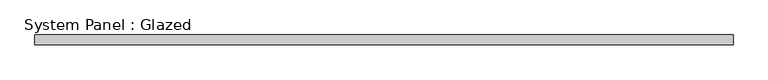
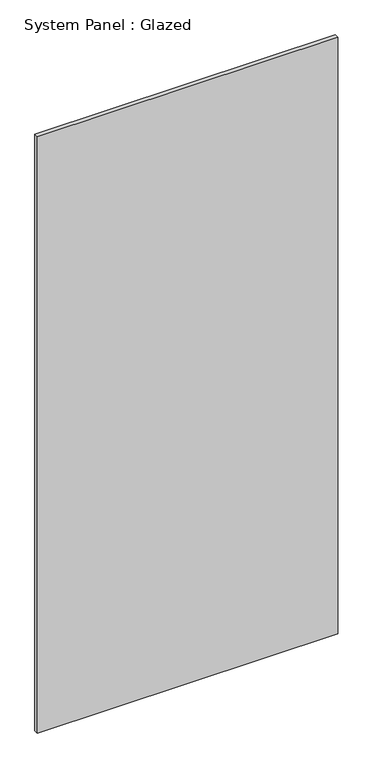
"""IFC4 building model written with IfcOpenShell, lengths in millimetres: plate geometry, System Panel : Glazed."""

from ifc_helpers import new_model, si_unit, origin, origin_with_axes, place, context, project, spatial, polyline, outline, extrude, source, transform, mapped, element, save


def system_panel_glazed_aacaf49b(model_context):
    return source(origin(), model_context, "Body", "SweptSolid", [
        extrude(outline(polyline([(904.9999998, 24.5), (-904.9999998, 24.5), (-904.9999998, 49.5), (904.9999998, 49.5), (904.9999998, 24.5)])), origin_with_axes(), (0.0, 0.0, 1.0), 3800.0),
    ])


if __name__ == "__main__":
    model = new_model("IFC4")
    model_context = context("Model", 3, world=origin())
    ifc_project = project(units=[si_unit("LENGTHUNIT", "METRE", prefix="MILLI")], contexts=[model_context])
    site = spatial("IfcSite", under=ifc_project)
    building = spatial("IfcBuilding", under=site)
    placement = place(None, origin())
    system_panel_glazed_shape = system_panel_glazed_aacaf49b(model_context)
    element("IfcPlate", 1, ObjectType="System Panel : Glazed", at=placement, inside=building, context=model_context, shape_type="MappedRepresentation", body=[
        mapped(system_panel_glazed_shape, transform((0.0, 0.0, 0.0), x_axis=(1.0, 0.0, 0.0), y_axis=(0.0, 1.0, 0.0), z_axis=(0.0, 0.0, 1.0))),
    ])
    save(model, "model.ifc")

# Revit data of these elements
# Type "System Panel : Glazed"
#   Construction Type Id = "GSP4R"
#   Analytic Construction = "1/8 in Pilkington single glazing"
#   Visual Light Transmittance = 0.9
#   Solar Heat Gain Coefficient = 0.86
#   Heat Transfer Coefficient (U) = 6.7069 W/(m²·K)
#   Define Thermal Properties by = 1
# Element 1 (IfcPlate, "System Panel : Glazed")
#   Materials on its faces: "Glass"
# Materials
#   "Glass": class "Glass", colour RGB 0 128 192, transparency 0.9, Description = "Soda Lime Glass", Cost = 0
